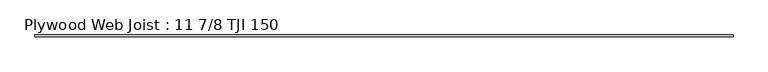
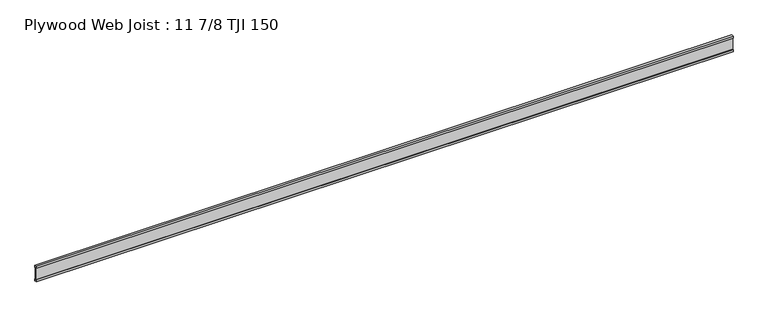
"""IFC4 building model written with IfcOpenShell, lengths in millimetres: beam geometry, Plywood Web Joist : 11 7/8 TJI 150."""

import ifcopenshell
import ifcopenshell.guid

model = None  # the IFC model being written
_history = None  # IfcOwnerHistory: only IFC2X3 demands one
_inside = {}  # id of a spatial element -> (the spatial element, [elements in it])
_under = {}  # id of a project, library or spatial element -> (it, [spatial elements below it])
_declared = {}  # id of a project -> (the project, [libraries it declares])
_typed = {}  # id of a type object -> (the type object, [elements of that type])
_made_of = {}  # id of a material, layer set ... -> (it, [elements and type objects made of it])


def new_model(schema):
    """Start an empty IFC model of exactly this schema.

    Asked for "IFC4X3", IfcOpenShell would pick the latest addendum, in which some entities
    have other attributes; the version numbers below select the first issue.
    IFC2X3 requires an IfcOwnerHistory on every rooted entity: one is made here for all.
    """
    global model, _history
    if schema == "IFC4X3":
        model = ifcopenshell.file(schema_version=(4, 3, 0, 0))
    else:
        model = ifcopenshell.file(schema=schema)
    _inside.clear()
    _under.clear()
    _declared.clear()
    _typed.clear()
    _made_of.clear()
    _history = None
    if model.schema == "IFC2X3":
        org = make("IfcOrganization", Name="unknown")
        user = make(
            "IfcPersonAndOrganization",
            ThePerson=make("IfcPerson", FamilyName="unknown"),
            TheOrganization=org,
        )
        app = make(
            "IfcApplication",
            ApplicationDeveloper=org,
            Version="unknown",
            ApplicationFullName="unknown",
            ApplicationIdentifier="unknown",
        )
        _history = make(
            "IfcOwnerHistory",
            OwningUser=user,
            OwningApplication=app,
            ChangeAction="ADDED",
            CreationDate=0,
        )
    return model


def make(cls, **values):
    """One entity of the class cls with the attributes given. An attribute that is None is left unset."""
    return model.create_entity(
        cls, **{name: value for name, value in values.items() if value is not None}
    )


def rooted(cls, **values):
    """An entity with a GlobalId (a new one), such as an element, a storey or a relation."""
    return make(cls, GlobalId=ifcopenshell.guid.new(), OwnerHistory=_history, **values)


def si_unit(unit_type, name, prefix=None):
    """IfcSIUnit, for example si_unit("LENGTHUNIT", "METRE", prefix="MILLI")."""
    return make("IfcSIUnit", UnitType=unit_type, Prefix=prefix, Name=name)


def assignment(units):
    """IfcUnitAssignment: the units of a project."""
    return None if units is None else make("IfcUnitAssignment", Units=units)


def point(xyz):
    """IfcCartesianPoint."""
    return None if xyz is None else make("IfcCartesianPoint", Coordinates=xyz)


def direction(xyz):
    """IfcDirection."""
    return None if xyz is None else make("IfcDirection", DirectionRatios=xyz)


def frame(location, z_axis=None, x_axis=None):
    """IfcAxis2Placement3D, a coordinate frame: its origin and axes. An axis left out is left unset."""
    return make(
        "IfcAxis2Placement3D",
        Location=point(location),
        Axis=direction(z_axis),
        RefDirection=direction(x_axis),
    )


def origin():
    """The frame at (0, 0, 0) with its axes left unset."""
    return frame((0.0, 0.0, 0.0))


def place(relative_to, where):
    """IfcLocalPlacement: puts the frame where relative to a parent placement (None: the world)."""
    return make(
        "IfcLocalPlacement", PlacementRelTo=relative_to, RelativePlacement=where
    )


def context(
    kind, dimensions, precision=None, world=None, true_north=None, identifier=None
):
    """IfcGeometricRepresentationContext, for example the 3D "Model" context."""
    return make(
        "IfcGeometricRepresentationContext",
        ContextIdentifier=identifier,
        ContextType=kind,
        CoordinateSpaceDimension=dimensions,
        Precision=precision,
        WorldCoordinateSystem=world,
        TrueNorth=true_north,
    )


def project(units=None, contexts=None):
    """IfcProject with its units and contexts."""
    return rooted(
        "IfcProject",
        Name="project",
        RepresentationContexts=contexts,
        UnitsInContext=assignment(units),
    )


def spatial(cls, under=None, at=None, **own):
    """A site, building, storey or space (cls), placed at a placement, below another one or the project."""
    s = rooted(cls, ObjectPlacement=at, **own)
    if under is not None:
        _under.setdefault(under.id(), (under, []))[1].append(s)
    return s


def polyline(points):
    """IfcPolyline through the points."""
    return make("IfcPolyline", Points=[point(p) for p in points])


def outline(outer, holes=None, kind="AREA"):
    """IfcArbitraryClosedProfileDef: a profile drawn as a closed curve; with holes, ...WithVoids."""
    if holes is None:
        return make("IfcArbitraryClosedProfileDef", ProfileType=kind, OuterCurve=outer)
    return make(
        "IfcArbitraryProfileDefWithVoids",
        ProfileType=kind,
        OuterCurve=outer,
        InnerCurves=holes,
    )


def extrude(swept, where, along, depth):
    """IfcExtrudedAreaSolid: the profile swept, set in the frame where, extruded along a direction by depth."""
    return make(
        "IfcExtrudedAreaSolid",
        SweptArea=swept,
        Position=where,
        ExtrudedDirection=direction(along),
        Depth=depth,
    )


def shape(context_of_items, identifier, shape_type, items):
    """IfcShapeRepresentation: the items that make up one representation, for example the "Body"."""
    return make(
        "IfcShapeRepresentation",
        ContextOfItems=context_of_items,
        RepresentationIdentifier=identifier,
        RepresentationType=shape_type,
        Items=items,
    )


def source(mapping_origin, context_of_items, identifier, shape_type, items):
    """IfcRepresentationMap: a shape defined once, which mapped items show again and again."""
    return make(
        "IfcRepresentationMap",
        MappingOrigin=mapping_origin,
        MappedRepresentation=shape(context_of_items, identifier, shape_type, items),
    )


def transform(
    local_origin,
    x_axis=None,
    y_axis=None,
    z_axis=None,
    scale=None,
    scale2=None,
    scale3=None,
    uniform=True,
):
    """IfcCartesianTransformationOperator3D, or its non-uniform kind. x_axis, y_axis, z_axis: its Axis1, 2, 3."""
    if uniform:
        return make(
            "IfcCartesianTransformationOperator3D",
            Axis1=direction(x_axis),
            Axis2=direction(y_axis),
            LocalOrigin=point(local_origin),
            Scale=scale,
            Axis3=direction(z_axis),
        )
    return make(
        "IfcCartesianTransformationOperator3DnonUniform",
        Axis1=direction(x_axis),
        Axis2=direction(y_axis),
        LocalOrigin=point(local_origin),
        Scale=scale,
        Axis3=direction(z_axis),
        Scale2=scale2,
        Scale3=scale3,
    )


def mapped(mapping_source, mapping_target):
    """IfcMappedItem: shows the shape of a source again, moved by a transform."""
    return make(
        "IfcMappedItem", MappingSource=mapping_source, MappingTarget=mapping_target
    )


def made_of(thing, what):
    """Note that an element or type object is made of a material, layer set ...; save() writes the relation."""
    if what is not None:
        _made_of.setdefault(what.id(), (what, []))[1].append(thing)
    return thing


def element(
    cls,
    number,
    at=None,
    inside=None,
    cuts=None,
    type_object=None,
    material=None,
    context=None,
    identifier="Body",
    shape_type=None,
    held_by="IfcProductDefinitionShape",
    body=None,
    shapes=None,
    **own,
):
    """One element of the class cls, such as IfcWall. Its Tag is "e" and its number.

    at: its placement. inside: the storey or other place that contains it. cuts: it is an
    opening in that element (IfcRelVoidsElement). A single representation is given by context,
    identifier, shape_type and body (its items); several are given by shapes. held_by: the class
    of the entity that holds the representations. save() writes the other relations.
    """
    e = rooted(cls, Tag="e%d" % number, ObjectPlacement=at, **own)
    if body is not None:
        shapes = [shape(context, identifier, shape_type, body)]
    if shapes is not None:
        e.Representation = make(held_by, Representations=shapes)
    if inside is not None:
        _inside.setdefault(inside.id(), (inside, []))[1].append(e)
    if cuts is not None:
        rooted(
            "IfcRelVoidsElement", RelatingBuildingElement=cuts, RelatedOpeningElement=e
        )
    if type_object is not None:
        _typed.setdefault(type_object.id(), (type_object, []))[1].append(e)
    return made_of(e, material)


def aggregate(whole, parts):
    """IfcRelAggregates: a whole, such as a stair, and the parts it consists of."""
    return rooted("IfcRelAggregates", RelatingObject=whole, RelatedObjects=parts)


def save(model, path):
    """Write the relations noted so far, then the file.

    IfcRelAggregates (storeys below a building ...), IfcRelContainedInSpatialStructure (elements
    in a storey), IfcRelDefinesByType, IfcRelAssociatesMaterial and IfcRelDeclares: one each for
    every whole, place, type object, material and project.
    """
    for whole, parts in _under.values():
        aggregate(whole, parts)
    for where, things in _inside.values():
        rooted(
            "IfcRelContainedInSpatialStructure",
            RelatedElements=things,
            RelatingStructure=where,
        )
    for kind, things in _typed.values():
        rooted("IfcRelDefinesByType", RelatedObjects=things, RelatingType=kind)
    for what, things in _made_of.values():
        rooted("IfcRelAssociatesMaterial", RelatedObjects=things, RelatingMaterial=what)
    for by, libraries in _declared.values():
        rooted("IfcRelDeclares", RelatingContext=by, RelatedDefinitions=libraries)
    model.write(path)


def plywood_web_joist_11_7_8_tji_150_6827b9fe(model_context):
    return source(origin(), model_context, "Body", "SweptSolid", [
        extrude(outline(polyline([(-19.05, 150.8125), (19.05, 150.8125), (19.05, 112.7125), (4.7625, 112.7125), (4.7625, 119.0625), (-4.7625, 119.0625), (-4.7625, 112.7125), (-19.05, 112.7125), (-19.05, 150.8125)])), frame((-6407.15, 0.0, 0.0), z_axis=(1.0, 0.0, 0.0), x_axis=(0.0, 1.0, 0.0)), (0.0, 0.0, 1.0), 12812.7125),
        extrude(outline(polyline([(19.05, -112.7125), (19.05, -150.8125), (-19.05, -150.8125), (-19.05, -112.7125), (-4.7625, -112.7125), (-4.7625, -118.3285374), (4.7625, -118.3285374), (4.7625, -112.7125), (19.05, -112.7125)])), frame((-6407.15, 0.0, 0.0), z_axis=(1.0, 0.0, 0.0), x_axis=(0.0, 1.0, 0.0)), (0.0, 0.0, 1.0), 12812.7125),
        extrude(outline(polyline([(6405.5625, 4.7625), (6405.5625, -4.7625), (-6407.15, -4.7625), (-6407.15, 4.7625), (6405.5625, 4.7625)])), frame((0.0, 0.0, -118.3285374), z_axis=(0.0, 0.0, 1.0), x_axis=(1.0, 0.0, 0.0)), (0.0, 0.0, 1.0), 237.3910374),
    ])


if __name__ == "__main__":
    model = new_model("IFC4")
    model_context = context("Model", 3, world=origin())
    ifc_project = project(units=[si_unit("LENGTHUNIT", "METRE", prefix="MILLI")], contexts=[model_context])
    site = spatial("IfcSite", under=ifc_project)
    building = spatial("IfcBuilding", under=site)
    placement = place(None, origin())
    plywood_web_joist_11_7_8_tji_150_shape = plywood_web_joist_11_7_8_tji_150_6827b9fe(model_context)
    element("IfcBeam", 1, ObjectType="Plywood Web Joist : 11 7/8 TJI 150", at=placement, inside=building, context=model_context, shape_type="MappedRepresentation", body=[
        mapped(plywood_web_joist_11_7_8_tji_150_shape, transform((0.0, 0.0, 0.0), x_axis=(1.0, 0.0, 0.0), y_axis=(0.0, 1.0, 0.0), z_axis=(0.0, 0.0, 1.0))),
    ])
    save(model, "model.ifc")

# Revit data of these elements
# Type "Plywood Web Joist : 11 7/8 TJI 150"
#   Assembly Code = "B10"
#   Cost = 17.5
#   Length [instance default] = 5' - 0"
#   b = 0' - 1 1/2"
#   d = 0' - 11 7/8"
#   Structural Material [instance default] = Softwood, Lumber
# Element 1 (IfcBeam, "Plywood Web Joist : 11 7/8 TJI 150")
#   Structural Material = Douglas Fir #2
#   Materials on its faces: "Douglas Fir #2"
# Materials
#   "Softwood, Lumber": class "Wood", colour RGB 223 192 134, transparency 0, Description = "Pinus Echinata", Cost = 0
#   "Douglas Fir #2": class "Wood", colour RGB 223 192 134, transparency 0, Description = "Pinus Echinata", Cost = 0
